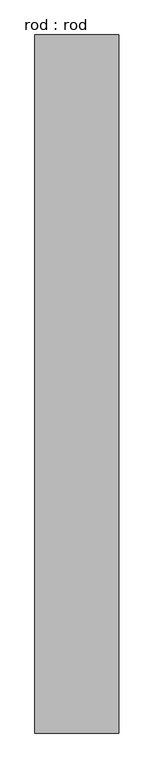
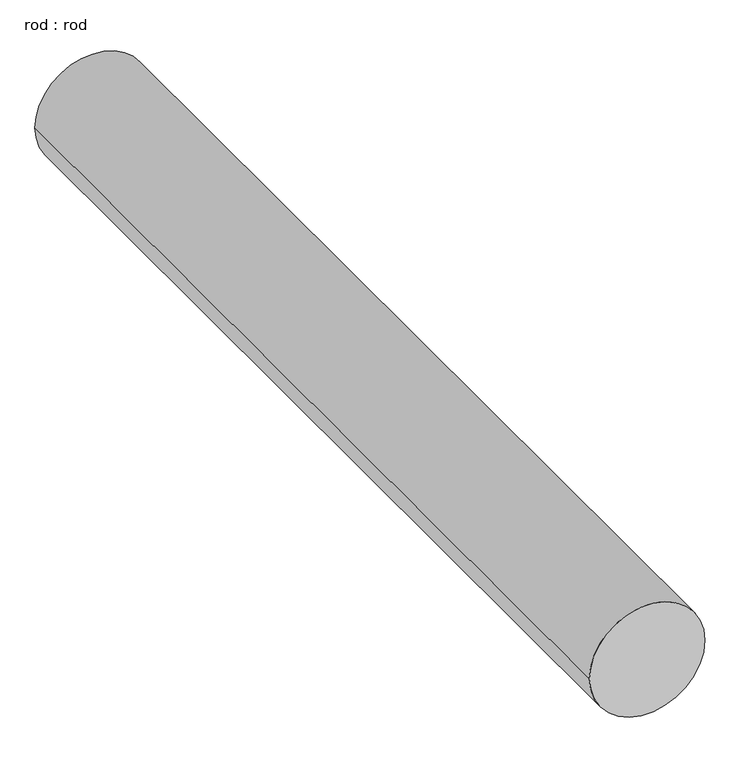
"""IFC4 building model written with IfcOpenShell, lengths in millimetres: proxy geometry, rod : rod."""

from ifc_helpers import new_model, si_unit, point, frame, frame_2d, origin, place, context, project, spatial, circle_curve, trimmed, segment, composite_curve, outline, extrude, source, transform, mapped, element, save


def rod_rod_e2998af1(model_context):
    return source(origin(), model_context, "Body", "SweptSolid", [
        extrude(outline(composite_curve([segment(trimmed(circle_curve(frame_2d((0.0108462, 0.0)), 200.0), [point((0.0108462, 200.0))], [point((0.0108462, -200.0))], False, "CARTESIAN"), True, "CONTINUOUS"), segment(trimmed(circle_curve(frame_2d((0.0108462, 0.0)), 200.0), [point((0.0108462, -200.0))], [point((0.0108462, 200.0))], False, "CARTESIAN"), True, "CONTINUOUS")], self_intersect=False)), frame((0.0, 2426.6571868, 0.0), z_axis=(0.0, 1.0, 0.0), x_axis=(0.0, 0.0, 1.0)), (0.0, 0.0, 1.0), 3332.1428571),
    ])


if __name__ == "__main__":
    model = new_model("IFC4")
    model_context = context("Model", 3, world=origin())
    ifc_project = project(units=[si_unit("LENGTHUNIT", "METRE", prefix="MILLI")], contexts=[model_context])
    site = spatial("IfcSite", under=ifc_project)
    building = spatial("IfcBuilding", under=site)
    placement = place(None, origin())
    rod_rod_shape = rod_rod_e2998af1(model_context)
    element("IfcBuildingElementProxy", 1, Name="rod : rod", ObjectType="rod : rod", at=placement, inside=building, context=model_context, shape_type="MappedRepresentation", body=[
        mapped(rod_rod_shape, transform((0.0, 0.0, 0.0), x_axis=(1.0, 0.0, 0.0), y_axis=(0.0, 1.0, 0.0), z_axis=(0.0, 0.0, 1.0))),
    ])
    save(model, "model.ifc")

# Revit data of these elements
# Type "rod : rod"
#   Default Elevation = 0
